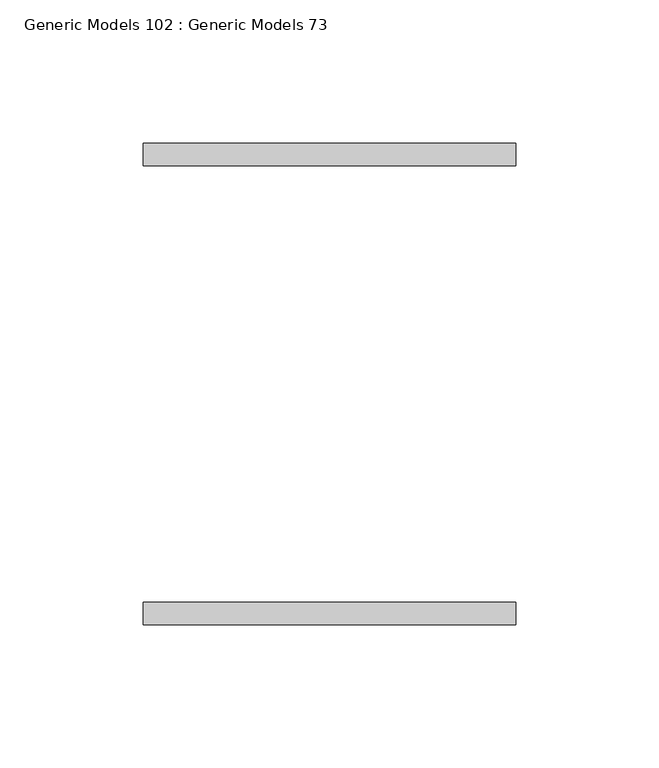
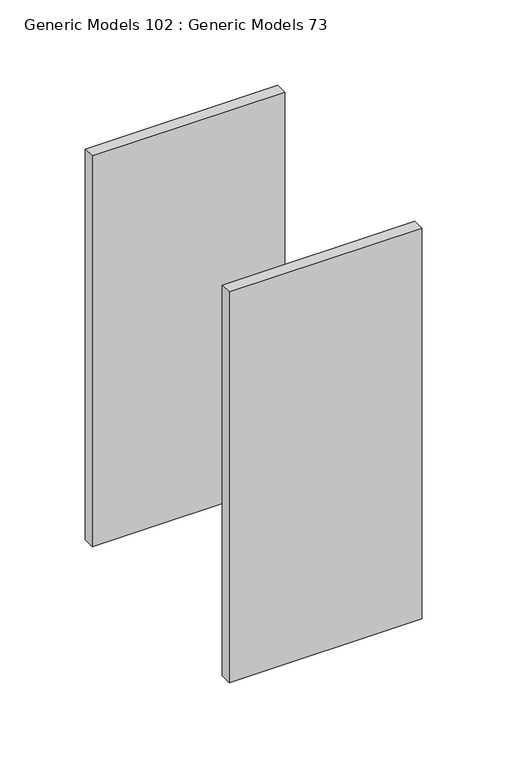
"""IFC4 building model written with IfcOpenShell, lengths in millimetres: proxy geometry, Generic Models 102 : Generic Models 73."""

from ifc_helpers import new_model, si_unit, frame, origin, place, context, project, spatial, polyline, outline, extrude, source, transform, mapped, element, save


def generic_models_102_generic_models_73_cec9b0b2(model_context):
    return source(origin(), model_context, "Body", "SweptSolid", [
        extrude(outline(polyline([(32040.4971032, 30858.4781612), (32040.4971032, 30850.5406612), (31910.3221032, 30850.5406612), (31910.3221032, 30858.4781612), (32040.4971032, 30858.4781612)])), frame((0.0, 0.0, 269146.3375), z_axis=(0.0, 0.0, 1.0), x_axis=(1.0, 0.0, 0.0)), (0.0, 0.0, 1.0), 279.4),
        extrude(outline(polyline([(32040.4971032, 30698.1406612), (32040.4971032, 30690.2031612), (31910.3221032, 30690.2031612), (31910.3221032, 30698.1406612), (32040.4971032, 30698.1406612)])), frame((0.0, 0.0, 269146.3375), z_axis=(0.0, 0.0, 1.0), x_axis=(1.0, 0.0, 0.0)), (0.0, 0.0, 1.0), 279.4),
    ])


if __name__ == "__main__":
    model = new_model("IFC4")
    model_context = context("Model", 3, world=origin())
    ifc_project = project(units=[si_unit("LENGTHUNIT", "METRE", prefix="MILLI")], contexts=[model_context])
    site = spatial("IfcSite", under=ifc_project)
    building = spatial("IfcBuilding", under=site)
    placement = place(None, origin())
    generic_models_102_generic_models_73_shape = generic_models_102_generic_models_73_cec9b0b2(model_context)
    element("IfcBuildingElementProxy", 1, Name="Generic Models 102 : Generic Models 73", ObjectType="Generic Models 102 : Generic Models 73", at=placement, inside=building, context=model_context, shape_type="MappedRepresentation", body=[
        mapped(generic_models_102_generic_models_73_shape, transform((0.0, 0.0, 0.0), x_axis=(1.0, 0.0, 0.0), y_axis=(0.0, 1.0, 0.0), z_axis=(0.0, 0.0, 1.0))),
    ])
    save(model, "model.ifc")

# Revit data of these elements
# Element 1 (IfcBuildingElementProxy, "Generic Models 102 : Generic Models 73")
#   Materials on its faces: "5/16 x 9 x 0'-11\" SIDE PLATES  CAP\nW/ 2 3/4\"DIA. THRU BOLTS"
# Materials
#   "5/16 x 9 x 0'-11\" SIDE PLATES  CAP\nW/ 2 3/4\"DIA. THRU BOLTS": class "Metal", colour RGB 199 199 199, transparency 0, Description = "Carbon steel", Cost = 0
